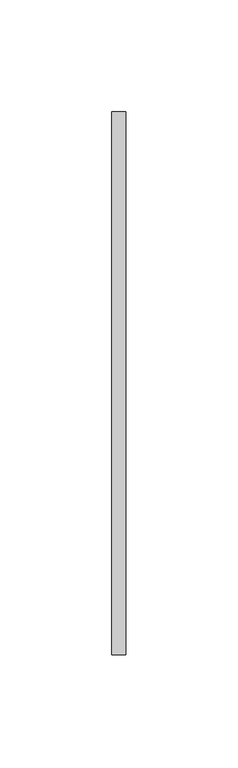
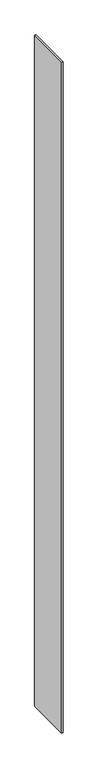
"""IFC4 building model written with IfcOpenShell, lengths in millimetres: proxy geometry, Inner panel1:Inner panel:306176:Inner panel:306176 : Inner panel1:Inner panel:306176:300391:Inner panel:306176:Inner panel:306176 : Inner panel1:Inner panel:306176:300391 : Inner panel1:Inner panel:306176:Inner panel:306176 : Inner panel1:Inner panel:306176:300391:6 : Inner panel1:Inner panel:306176:Inner panel:306176 : Inner panel1:Inner panel:306176:300391:Inner panel:306176:Inner panel:306176 : Inner panel1:Inner panel:306176:300391 : Inner panel1:Inner panel:306176:Inner panel:306176 : Inner panel1:Inner panel:306176:300391:300168."""

import ifcopenshell
import ifcopenshell.guid

model = None  # the IFC model being written
_history = None  # IfcOwnerHistory: only IFC2X3 demands one
_inside = {}  # id of a spatial element -> (the spatial element, [elements in it])
_under = {}  # id of a project, library or spatial element -> (it, [spatial elements below it])
_declared = {}  # id of a project -> (the project, [libraries it declares])
_typed = {}  # id of a type object -> (the type object, [elements of that type])
_made_of = {}  # id of a material, layer set ... -> (it, [elements and type objects made of it])


def new_model(schema):
    """Start an empty IFC model of exactly this schema.

    Asked for "IFC4X3", IfcOpenShell would pick the latest addendum, in which some entities
    have other attributes; the version numbers below select the first issue.
    IFC2X3 requires an IfcOwnerHistory on every rooted entity: one is made here for all.
    """
    global model, _history
    if schema == "IFC4X3":
        model = ifcopenshell.file(schema_version=(4, 3, 0, 0))
    else:
        model = ifcopenshell.file(schema=schema)
    _inside.clear()
    _under.clear()
    _declared.clear()
    _typed.clear()
    _made_of.clear()
    _history = None
    if model.schema == "IFC2X3":
        org = make("IfcOrganization", Name="unknown")
        user = make(
            "IfcPersonAndOrganization",
            ThePerson=make("IfcPerson", FamilyName="unknown"),
            TheOrganization=org,
        )
        app = make(
            "IfcApplication",
            ApplicationDeveloper=org,
            Version="unknown",
            ApplicationFullName="unknown",
            ApplicationIdentifier="unknown",
        )
        _history = make(
            "IfcOwnerHistory",
            OwningUser=user,
            OwningApplication=app,
            ChangeAction="ADDED",
            CreationDate=0,
        )
    return model


def make(cls, **values):
    """One entity of the class cls with the attributes given. An attribute that is None is left unset."""
    return model.create_entity(
        cls, **{name: value for name, value in values.items() if value is not None}
    )


def rooted(cls, **values):
    """An entity with a GlobalId (a new one), such as an element, a storey or a relation."""
    return make(cls, GlobalId=ifcopenshell.guid.new(), OwnerHistory=_history, **values)


def si_unit(unit_type, name, prefix=None):
    """IfcSIUnit, for example si_unit("LENGTHUNIT", "METRE", prefix="MILLI")."""
    return make("IfcSIUnit", UnitType=unit_type, Prefix=prefix, Name=name)


def assignment(units):
    """IfcUnitAssignment: the units of a project."""
    return None if units is None else make("IfcUnitAssignment", Units=units)


def point(xyz):
    """IfcCartesianPoint."""
    return None if xyz is None else make("IfcCartesianPoint", Coordinates=xyz)


def direction(xyz):
    """IfcDirection."""
    return None if xyz is None else make("IfcDirection", DirectionRatios=xyz)


def frame(location, z_axis=None, x_axis=None):
    """IfcAxis2Placement3D, a coordinate frame: its origin and axes. An axis left out is left unset."""
    return make(
        "IfcAxis2Placement3D",
        Location=point(location),
        Axis=direction(z_axis),
        RefDirection=direction(x_axis),
    )


def origin():
    """The frame at (0, 0, 0) with its axes left unset."""
    return frame((0.0, 0.0, 0.0))


def place(relative_to, where):
    """IfcLocalPlacement: puts the frame where relative to a parent placement (None: the world)."""
    return make(
        "IfcLocalPlacement", PlacementRelTo=relative_to, RelativePlacement=where
    )


def context(
    kind, dimensions, precision=None, world=None, true_north=None, identifier=None
):
    """IfcGeometricRepresentationContext, for example the 3D "Model" context."""
    return make(
        "IfcGeometricRepresentationContext",
        ContextIdentifier=identifier,
        ContextType=kind,
        CoordinateSpaceDimension=dimensions,
        Precision=precision,
        WorldCoordinateSystem=world,
        TrueNorth=true_north,
    )


def project(units=None, contexts=None):
    """IfcProject with its units and contexts."""
    return rooted(
        "IfcProject",
        Name="project",
        RepresentationContexts=contexts,
        UnitsInContext=assignment(units),
    )


def spatial(cls, under=None, at=None, **own):
    """A site, building, storey or space (cls), placed at a placement, below another one or the project."""
    s = rooted(cls, ObjectPlacement=at, **own)
    if under is not None:
        _under.setdefault(under.id(), (under, []))[1].append(s)
    return s


def polyline(points):
    """IfcPolyline through the points."""
    return make("IfcPolyline", Points=[point(p) for p in points])


def outline(outer, holes=None, kind="AREA"):
    """IfcArbitraryClosedProfileDef: a profile drawn as a closed curve; with holes, ...WithVoids."""
    if holes is None:
        return make("IfcArbitraryClosedProfileDef", ProfileType=kind, OuterCurve=outer)
    return make(
        "IfcArbitraryProfileDefWithVoids",
        ProfileType=kind,
        OuterCurve=outer,
        InnerCurves=holes,
    )


def extrude(swept, where, along, depth):
    """IfcExtrudedAreaSolid: the profile swept, set in the frame where, extruded along a direction by depth."""
    return make(
        "IfcExtrudedAreaSolid",
        SweptArea=swept,
        Position=where,
        ExtrudedDirection=direction(along),
        Depth=depth,
    )


def shape(context_of_items, identifier, shape_type, items):
    """IfcShapeRepresentation: the items that make up one representation, for example the "Body"."""
    return make(
        "IfcShapeRepresentation",
        ContextOfItems=context_of_items,
        RepresentationIdentifier=identifier,
        RepresentationType=shape_type,
        Items=items,
    )


def source(mapping_origin, context_of_items, identifier, shape_type, items):
    """IfcRepresentationMap: a shape defined once, which mapped items show again and again."""
    return make(
        "IfcRepresentationMap",
        MappingOrigin=mapping_origin,
        MappedRepresentation=shape(context_of_items, identifier, shape_type, items),
    )


def transform(
    local_origin,
    x_axis=None,
    y_axis=None,
    z_axis=None,
    scale=None,
    scale2=None,
    scale3=None,
    uniform=True,
):
    """IfcCartesianTransformationOperator3D, or its non-uniform kind. x_axis, y_axis, z_axis: its Axis1, 2, 3."""
    if uniform:
        return make(
            "IfcCartesianTransformationOperator3D",
            Axis1=direction(x_axis),
            Axis2=direction(y_axis),
            LocalOrigin=point(local_origin),
            Scale=scale,
            Axis3=direction(z_axis),
        )
    return make(
        "IfcCartesianTransformationOperator3DnonUniform",
        Axis1=direction(x_axis),
        Axis2=direction(y_axis),
        LocalOrigin=point(local_origin),
        Scale=scale,
        Axis3=direction(z_axis),
        Scale2=scale2,
        Scale3=scale3,
    )


def mapped(mapping_source, mapping_target):
    """IfcMappedItem: shows the shape of a source again, moved by a transform."""
    return make(
        "IfcMappedItem", MappingSource=mapping_source, MappingTarget=mapping_target
    )


def made_of(thing, what):
    """Note that an element or type object is made of a material, layer set ...; save() writes the relation."""
    if what is not None:
        _made_of.setdefault(what.id(), (what, []))[1].append(thing)
    return thing


def element(
    cls,
    number,
    at=None,
    inside=None,
    cuts=None,
    type_object=None,
    material=None,
    context=None,
    identifier="Body",
    shape_type=None,
    held_by="IfcProductDefinitionShape",
    body=None,
    shapes=None,
    **own,
):
    """One element of the class cls, such as IfcWall. Its Tag is "e" and its number.

    at: its placement. inside: the storey or other place that contains it. cuts: it is an
    opening in that element (IfcRelVoidsElement). A single representation is given by context,
    identifier, shape_type and body (its items); several are given by shapes. held_by: the class
    of the entity that holds the representations. save() writes the other relations.
    """
    e = rooted(cls, Tag="e%d" % number, ObjectPlacement=at, **own)
    if body is not None:
        shapes = [shape(context, identifier, shape_type, body)]
    if shapes is not None:
        e.Representation = make(held_by, Representations=shapes)
    if inside is not None:
        _inside.setdefault(inside.id(), (inside, []))[1].append(e)
    if cuts is not None:
        rooted(
            "IfcRelVoidsElement", RelatingBuildingElement=cuts, RelatedOpeningElement=e
        )
    if type_object is not None:
        _typed.setdefault(type_object.id(), (type_object, []))[1].append(e)
    return made_of(e, material)


def aggregate(whole, parts):
    """IfcRelAggregates: a whole, such as a stair, and the parts it consists of."""
    return rooted("IfcRelAggregates", RelatingObject=whole, RelatedObjects=parts)


def save(model, path):
    """Write the relations noted so far, then the file.

    IfcRelAggregates (storeys below a building ...), IfcRelContainedInSpatialStructure (elements
    in a storey), IfcRelDefinesByType, IfcRelAssociatesMaterial and IfcRelDeclares: one each for
    every whole, place, type object, material and project.
    """
    for whole, parts in _under.values():
        aggregate(whole, parts)
    for where, things in _inside.values():
        rooted(
            "IfcRelContainedInSpatialStructure",
            RelatedElements=things,
            RelatingStructure=where,
        )
    for kind, things in _typed.values():
        rooted("IfcRelDefinesByType", RelatedObjects=things, RelatingType=kind)
    for what, things in _made_of.values():
        rooted("IfcRelAssociatesMaterial", RelatedObjects=things, RelatingMaterial=what)
    for by, libraries in _declared.values():
        rooted("IfcRelDeclares", RelatingContext=by, RelatedDefinitions=libraries)
    model.write(path)


def generic_models_2a76a65d(model_context):
    return source(origin(), model_context, "Body", "SweptSolid", [
        extrude(outline(polyline([(596209.8242239, -579014.9788841), (596209.8242239, -578772.0913841), (596216.1742239, -578772.0913841), (596216.1742239, -579014.9788841), (596209.8242239, -579014.9788841)])), frame((0.0, 0.0, 25.4), z_axis=(0.0, 0.0, 1.0), x_axis=(1.0, 0.0, 0.0)), (0.0, 0.0, 1.0), 3689.35),
    ])


if __name__ == "__main__":
    model = new_model("IFC4")
    model_context = context("Model", 3, world=origin())
    ifc_project = project(units=[si_unit("LENGTHUNIT", "METRE", prefix="MILLI")], contexts=[model_context])
    site = spatial("IfcSite", under=ifc_project)
    building = spatial("IfcBuilding", under=site)
    placement = place(None, origin())
    generic_models_shape = generic_models_2a76a65d(model_context)
    element("IfcBuildingElementProxy", 1, Name="Inner panel1:Inner panel:306176:Inner panel:306176 : Inner panel1:Inner panel:306176:300391:Inner panel:306176:Inner panel:306176 : Inner panel1:Inner panel:306176:300391 : Inner panel1:Inner panel:306176:Inner panel:306176 : Inner panel1:Inner panel:306176:300391:6 : Inner panel1:Inner panel:306176:Inner panel:306176 : Inner panel1:Inner panel:306176:300391:Inner panel:306176:Inner panel:306176 : Inner panel1:Inner panel:306176:300391 : Inner panel1:Inner panel:306176:Inner panel:306176 : Inner panel1:Inner panel:306176:300391:300168", ObjectType="Inner panel1:Inner panel:306176:Inner panel:306176 : Inner panel1:Inner panel:306176:300391:Inner panel:306176:Inner panel:306176 : Inner panel1:Inner panel:306176:300391 : Inner panel1:Inner panel:306176:Inner panel:306176 : Inner panel1:Inner panel:306176:300391:6 : Inner panel1:Inner panel:306176:Inner panel:306176 : Inner panel1:Inner panel:306176:300391:Inner panel:306176:Inner panel:306176 : Inner panel1:Inner panel:306176:300391 : Inner panel1:Inner panel:306176:Inner panel:306176 : Inner panel1:Inner panel:306176:300391:300168", at=placement, inside=building, context=model_context, shape_type="MappedRepresentation", body=[
        mapped(generic_models_shape, transform((0.0, 0.0, 0.0), x_axis=(1.0, 0.0, 0.0), y_axis=(0.0, 1.0, 0.0), z_axis=(0.0, 0.0, 1.0))),
    ])
    save(model, "model.ifc")

# Revit data of these elements
# Type "Inner panel1:Inner panel:306176:Inner panel:306176 : Inner panel1:Inner panel:306176:300391:Inner panel:306176:Inner panel:306176 : Inner panel1:Inner panel:306176:300391 : Inner panel1:Inner panel:306176:Inner panel:306176 : Inner panel1:Inner panel:306176:300391:6 : Inner panel1:Inner panel:306176:Inner panel:306176 : Inner panel1:Inner panel:306176:300391:Inner panel:306176:Inner panel:306176 : Inner panel1:Inner panel:306176:300391 : Inner panel1:Inner panel:306176:Inner panel:306176 : Inner panel1:Inner panel:306176:300391:300168"
#   NameOverride = "Inner panel1:Inner panel:306176:Inner panel:306176 : Inner panel1:Inner panel:306176:300391:Inner panel:306176:Inner panel:306176 : Inner panel1:Inner panel:306176:300391 : Inner panel1:Inner panel:306176:Inner panel:306176 : Inner panel1:Inner panel:306176:300391:300168"
#   ObjectTypeOverride = "Inner panel:306176:Inner panel:306176 : Inner panel1:Inner panel:306176:300391 : Inner panel1:Inner panel:306176:Inner panel:306176 : Inner panel1:Inner panel:306176:300391"
#   Reference = "Inner panel"
#   Tag = "300168"
# Element 1 (IfcBuildingElementProxy, "Inner panel1:Inner panel:306176:Inner panel:306176 : Inner panel1:Inner panel:306176:300391:Inner panel:306176:Inner panel:306176 : Inner panel1:Inner panel:306176:300391 : Inner panel1:Inner panel:306176:Inner panel:306176 : Inner panel1:Inner panel:306176:300391:6 : Inner panel1:Inner panel:306176:Inner panel:306176 : Inner panel1:Inner panel:306176:300391:Inner panel:306176:Inner panel:306176 : Inner panel1:Inner panel:306176:300391 : Inner panel1:Inner panel:306176:Inner panel:306176 : Inner panel1:Inner panel:306176:300391:300168")
#   Materials on its faces: "CERAMIC TILE"
# Materials
#   "CERAMIC TILE": class "Generic", colour RGB 87 103 117, transparency 0, Cost = 0
